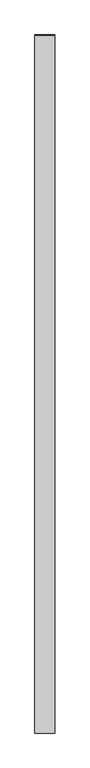
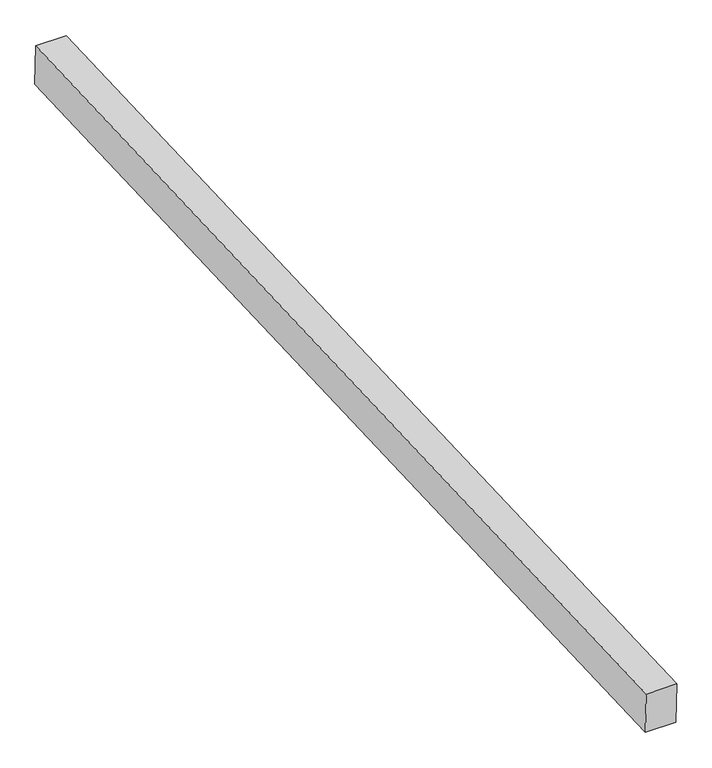
"""IFC4 building model written with IfcOpenShell, lengths in millimetres: proxy geometry, Generic Models 7:Generic Models 1:8:Generic Models 1:8 : Generic Models 7:Generic Models 1:337419:26 : Generic Models 7:Generic Models 1:8:Generic Models 1:8 : Generic Models 7:Generic Models 1:337419:315935."""

from ifc_helpers import new_model, si_unit, frame, origin, place, context, project, spatial, polyline, outline, extrude, source, transform, mapped, element, save


def generic_models_f91a96e2(model_context):
    return source(origin(), model_context, "Body", "SweptSolid", [
        extrude(outline(polyline([(-569809.5331552, 8697.9424054), (-564936.6102609, 8900.9808594), (-564929.0433392, 8710.6308549), (-569801.6025364, 8507.607555), (-569809.5331552, 8697.9424054)])), frame((596116.1617243, 0.0, 0.0), z_axis=(1.0, 0.0, 0.0), x_axis=(0.0, 1.0, 0.0)), (0.0, 0.0, 1.0), 139.7),
    ])


if __name__ == "__main__":
    model = new_model("IFC4")
    model_context = context("Model", 3, world=origin())
    ifc_project = project(units=[si_unit("LENGTHUNIT", "METRE", prefix="MILLI")], contexts=[model_context])
    site = spatial("IfcSite", under=ifc_project)
    building = spatial("IfcBuilding", under=site)
    placement = place(None, origin())
    generic_models_shape = generic_models_f91a96e2(model_context)
    element("IfcBuildingElementProxy", 1, Name="Generic Models 7:Generic Models 1:8:Generic Models 1:8 : Generic Models 7:Generic Models 1:337419:26 : Generic Models 7:Generic Models 1:8:Generic Models 1:8 : Generic Models 7:Generic Models 1:337419:315935", ObjectType="Generic Models 7:Generic Models 1:8:Generic Models 1:8 : Generic Models 7:Generic Models 1:337419:26 : Generic Models 7:Generic Models 1:8:Generic Models 1:8 : Generic Models 7:Generic Models 1:337419:315935", at=placement, inside=building, context=model_context, shape_type="MappedRepresentation", body=[
        mapped(generic_models_shape, transform((0.0, 0.0, 0.0), x_axis=(1.0, 0.0, 0.0), y_axis=(0.0, 1.0, 0.0), z_axis=(0.0, 0.0, 1.0))),
    ])
    save(model, "model.ifc")

# Revit data of these elements
# Type "Generic Models 7:Generic Models 1:8:Generic Models 1:8 : Generic Models 7:Generic Models 1:337419:26 : Generic Models 7:Generic Models 1:8:Generic Models 1:8 : Generic Models 7:Generic Models 1:337419:315935"
#   NameOverride = "Generic Models 7:Generic Models 1:8:Generic Models 1:8 : Generic Models 7:Generic Models 1:337419:315935"
#   ObjectTypeOverride = "Generic Models 1:8 : Generic Models 7:Generic Models 1:337419"
#   Reference = "Generic Models 1"
#   Tag = "315935"
# Element 1 (IfcBuildingElementProxy, "Generic Models 7:Generic Models 1:8:Generic Models 1:8 : Generic Models 7:Generic Models 1:337419:26 : Generic Models 7:Generic Models 1:8:Generic Models 1:8 : Generic Models 7:Generic Models 1:337419:315935")
#   Materials on its faces: "5 1/2\" X 7 1/2\" EXTERIOR GRADE GLULAM BEAMS"
# Materials
#   "5 1/2\" X 7 1/2\" EXTERIOR GRADE GLULAM BEAMS": class "Wood", colour RGB 183 134 68, transparency 0, Keynote = "M06181300.01", Description = "Pinus Echinata", Cost = 0
